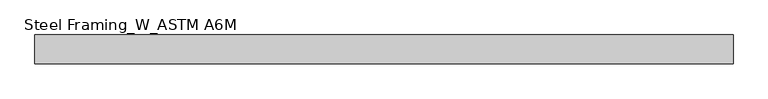
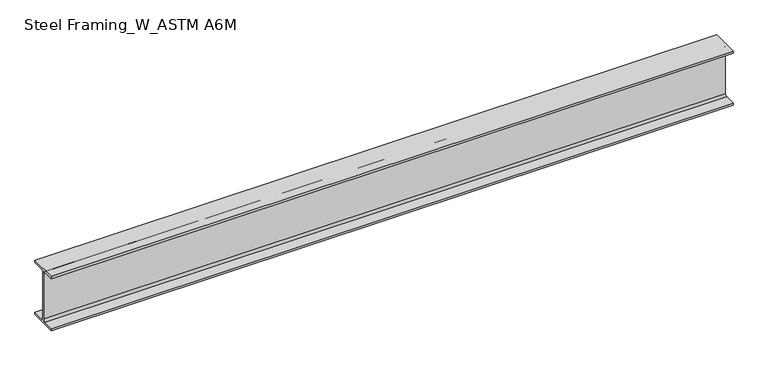
"""IFC4 building model written with IfcOpenShell, lengths in millimetres: beam geometry, Steel Framing_W_ASTM A6M : H_SB_AR_S02_W200x22.5_J1."""

from ifc_helpers import new_model, si_unit, point, frame, frame_2d, origin, place, context, project, spatial, polyline, circle_curve, trimmed, segment, composite_curve, outline, extrude, source, transform, mapped, element, save


def steel_framing_w_astm_a6m_a0e8152a(model_context):
    return source(origin(), model_context, "Body", "SweptSolid", [
        extrude(outline(composite_curve([segment(polyline([(51.0, -95.0), (51.0, -103.0), (-51.0, -103.0), (-51.0, -95.0), (-10.71, -95.0)]), True, "CONTINUOUS"), segment(trimmed(circle_curve(frame_2d((-10.71, -87.4)), 7.6), [point((-10.71, -95.0))], [point((-3.11, -87.4))], True, "CARTESIAN"), True, "CONTINUOUS"), segment(polyline([(-3.11, -87.4), (-3.11, 87.4)]), True, "CONTINUOUS"), segment(trimmed(circle_curve(frame_2d((-10.71, 87.4)), 7.6), [point((-3.11, 87.4))], [point((-10.71, 95.0))], True, "CARTESIAN"), True, "CONTINUOUS"), segment(polyline([(-10.71, 95.0), (-51.0, 95.0), (-51.0, 103.0), (51.0, 103.0), (51.0, 95.0), (10.71, 95.0)]), True, "CONTINUOUS"), segment(trimmed(circle_curve(frame_2d((10.71, 87.4)), 7.6), [point((10.71, 95.0))], [point((3.11, 87.4))], True, "CARTESIAN"), True, "CONTINUOUS"), segment(polyline([(3.11, 87.4), (3.11, -87.4)]), True, "CONTINUOUS"), segment(trimmed(circle_curve(frame_2d((10.71, -87.4)), 7.6), [point((3.11, -87.4))], [point((10.71, -95.0))], True, "CARTESIAN"), True, "CONTINUOUS"), segment(polyline([(10.71, -95.0), (51.0, -95.0)]), True, "CONTINUOUS")], self_intersect=False)), frame((-1255.3, 0.0, 0.0), z_axis=(1.0, 0.0, 0.0), x_axis=(0.0, 1.0, 0.0)), (0.0, 0.0, 1.0), 2450.6),
    ])


if __name__ == "__main__":
    model = new_model("IFC4")
    model_context = context("Model", 3, world=origin())
    ifc_project = project(units=[si_unit("LENGTHUNIT", "METRE", prefix="MILLI")], contexts=[model_context])
    site = spatial("IfcSite", under=ifc_project)
    building = spatial("IfcBuilding", under=site)
    placement = place(None, origin())
    steel_framing_w_astm_a6m_shape = steel_framing_w_astm_a6m_a0e8152a(model_context)
    element("IfcBeam", 1, ObjectType="Steel Framing_W_ASTM A6M : H_SB_AR_S02_W200x22.5_J1", at=placement, inside=building, context=model_context, shape_type="MappedRepresentation", body=[
        mapped(steel_framing_w_astm_a6m_shape, transform((0.0, 0.0, 0.0), x_axis=(1.0, 0.0, 0.0), y_axis=(0.0, 1.0, 0.0), z_axis=(0.0, 0.0, 1.0))),
    ])
    save(model, "model.ifc")

# Revit data of these elements
# Type "Steel Framing_W_ASTM A6M : H_SB_AR_S02_W200x22.5_J1"
#   Section Name Key = "W8x15"
#   Width = 10.2 cm
#   Web Thickness = 0.622 cm
#   Web Fillet = 0.76 cm
#   Warping Constant = 13900.0 cm⁶
#   Torsional Moment of Inertia = 5.70 cm⁴
#   Section Area = 28.6 cm²
#   Plastic Modulus weak axis = 43.8 cm³
#   Plastic Modulus strong axis = 223.0 cm³
#   Perimeter = 0.795 m²/m
#   Nominal Weight = 22.50 kgf/m
#   Moment of Inertia weak axis = 142.00 cm⁴
#   Moment of Inertia strong axis = 2000.00 cm⁴
#   Height = 20.6 cm
#   Flange Thickness = 0.8 cm
#   Elastic Modulus weak axis = 27.9 cm³
#   Elastic Modulus strong axis = 193.0 cm³
#   Centroid Vertical = 10.3 cm
#   Centroid Horizontal = 5.1 cm
#   Length [instance default] = 1500 mm
#   Structural Material [instance default] = Steel, 45-345
#   Bolt Spacing = 0
#   Assembly Code = ""
# Element 1 (IfcBeam, "Steel Framing_W_ASTM A6M : H_SB_AR_S02_W200x22.5_J1")
#   Materials on its faces: "Steel, 45-345"
# Materials
#   "Steel, 45-345": class "Metal", colour RGB 189 187 185, transparency 0, Description = "Steel 345 MPa", Cost = 0
